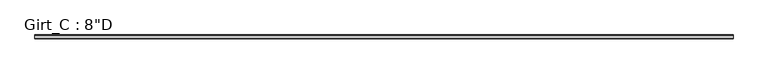
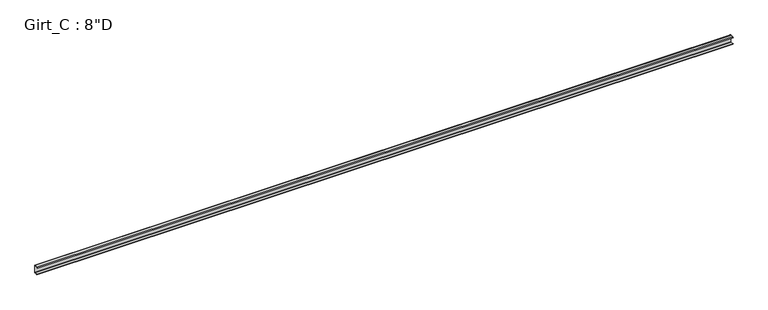
"""IFC4 building model written with IfcOpenShell, lengths in millimetres: beam geometry."""

from ifc_helpers import new_model, si_unit, point, frame, frame_2d, origin, place, context, project, spatial, polyline, circle_curve, trimmed, segment, composite_curve, outline, extrude, source, transform, mapped, element, save


def beam_336070c1(model_context):
    return source(origin(), model_context, "Body", "SweptSolid", [
        extrude(outline(composite_curve([segment(polyline([(-87.5109375, 101.6), (-3.3734375, 101.6)]), True, "CONTINUOUS"), segment(trimmed(circle_curve(frame_2d((-3.3734375, 96.8375)), 4.7625), [point((-3.3734375, 101.6))], [point((1.3890625, 96.8375))], False, "CARTESIAN"), True, "CONTINUOUS"), segment(polyline([(1.3890625, 96.8375), (1.3890625, -96.8375)]), True, "CONTINUOUS"), segment(trimmed(circle_curve(frame_2d((-3.3734375, -96.8375)), 4.7625), [point((1.3890625, -96.8375))], [point((-3.3734375, -101.6))], False, "CARTESIAN"), True, "CONTINUOUS"), segment(polyline([(-3.3734375, -101.6), (-87.5109375, -101.6), (-99.7792647, -86.979177), (-97.6510975, -85.1934327), (-86.2154765, -98.821875), (-3.2694106, -98.821875)]), True, "CONTINUOUS"), segment(trimmed(circle_curve(frame_2d((-3.3748024, -96.8389339)), 1.9857399), [point((-3.2694106, -98.821875))], [point((-1.3890625, -96.8389339))], True, "CARTESIAN"), True, "CONTINUOUS"), segment(polyline([(-1.3890625, -96.8389339), (-1.3890625, 96.8381931)]), True, "CONTINUOUS"), segment(trimmed(circle_curve(frame_2d((-3.3741066, 96.8381931)), 1.9850441), [point((-1.3890625, 96.8381931))], [point((-3.3005807, 98.821875))], True, "CARTESIAN"), True, "CONTINUOUS"), segment(polyline([(-3.3005807, 98.821875), (-86.2154765, 98.821875), (-97.6278742, 85.221109), (-99.7560415, 87.0068534), (-87.5109375, 101.6)]), True, "CONTINUOUS")], self_intersect=False)), frame((-9290.05, 0.0, 0.0), z_axis=(1.0, 0.0, 0.0), x_axis=(0.0, 1.0, 0.0)), (0.0, 0.0, 1.0), 18580.1),
    ])


if __name__ == "__main__":
    model = new_model("IFC4")
    model_context = context("Model", 3, world=origin())
    ifc_project = project(units=[si_unit("LENGTHUNIT", "METRE", prefix="MILLI")], contexts=[model_context])
    site = spatial("IfcSite", under=ifc_project)
    building = spatial("IfcBuilding", under=site)
    placement = place(None, origin())
    beam_shape = beam_336070c1(model_context)
    element("IfcBeam", 1, ObjectType="Girt_C : 8\"D", at=placement, inside=building, context=model_context, shape_type="MappedRepresentation", body=[
        mapped(beam_shape, transform((0.0, 0.0, 0.0), x_axis=(1.0, 0.0, 0.0), y_axis=(0.0, 1.0, 0.0), z_axis=(0.0, 0.0, 1.0))),
    ])
    save(model, "model.ifc")

# Revit data of these elements
# Type "Girt_C : 8\"D"
#   half leg = 0' - 1 3/4"
#   Web_Thickness = 0' - 0 7/64"
#   Length [instance default] = 10' - 0"
#   Leg_1 = 0' - 3 1/2"
#   Height = 0' - 8"
#   Structural Material [instance default] = none
# Element 1 (IfcBeam, "Girt_C : 8\"D")
#   Structural Material = GALVANIZED 'CEE' SECTION (8.0x3.5C - SEE STRUCT. DWGS)
#   Materials on its faces: "GALVANIZED 'CEE' SECTION (8.0x3.5C - SEE STRUCT. DWGS)"
# Materials
#   "GALVANIZED 'CEE' SECTION (8.0x3.5C - SEE STRUCT. DWGS)": class "Metal", colour RGB 137 146 153, transparency 0, Description = "Steel, mill finish", Cost = 0
